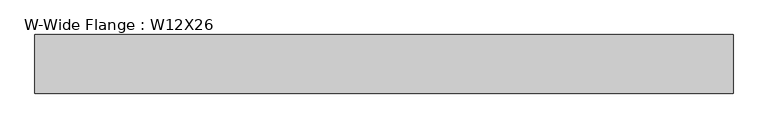
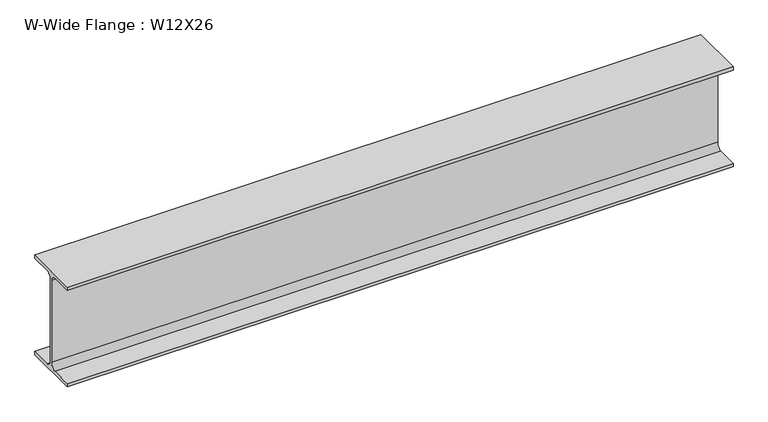
"""IFC4 building model written with IfcOpenShell, lengths in millimetres: beam geometry, W-Wide Flange : W12X26."""

from ifc_helpers import new_model, si_unit, point, frame, frame_2d, origin, place, context, project, spatial, polyline, circle_curve, trimmed, segment, composite_curve, outline, extrude, source, transform, mapped, element, save


def w_wide_flange_w12x26_057477a8(model_context):
    return source(origin(), model_context, "Body", "SweptSolid", [
        extrude(outline(composite_curve([segment(polyline([(-82.4011719, -145.5539063), (-20.2902344, -145.5539063)]), True, "CONTINUOUS"), segment(trimmed(circle_curve(frame_2d((-20.2902344, -128.190625)), 17.3632812), [point((-20.2902344, -145.5539063))], [point((-2.9269531, -128.190625))], True, "CARTESIAN"), True, "CONTINUOUS"), segment(polyline([(-2.9269531, -128.190625), (-2.9269531, 128.190625)]), True, "CONTINUOUS"), segment(trimmed(circle_curve(frame_2d((-20.2902344, 128.190625)), 17.3632812), [point((-2.9269531, 128.190625))], [point((-20.2902344, 145.5539062))], True, "CARTESIAN"), True, "CONTINUOUS"), segment(polyline([(-20.2902344, 145.5539062), (-82.4011719, 145.5539062), (-82.4011719, 155.178125), (82.4011719, 155.178125), (82.4011719, 145.5539062), (20.2902344, 145.5539062)]), True, "CONTINUOUS"), segment(trimmed(circle_curve(frame_2d((20.2902344, 128.190625)), 17.3632812), [point((20.2902344, 145.5539062))], [point((2.9269531, 128.190625))], True, "CARTESIAN"), True, "CONTINUOUS"), segment(polyline([(2.9269531, 128.190625), (2.9269531, -128.190625)]), True, "CONTINUOUS"), segment(trimmed(circle_curve(frame_2d((20.2902344, -128.190625)), 17.3632812), [point((2.9269531, -128.190625))], [point((20.2902344, -145.5539063))], True, "CARTESIAN"), True, "CONTINUOUS"), segment(polyline([(20.2902344, -145.5539063), (82.4011719, -145.5539063), (82.4011719, -155.178125), (-82.4011719, -155.178125), (-82.4011719, -145.5539063)]), True, "CONTINUOUS")], self_intersect=False)), frame((-984.25, 0.0, 0.0), z_axis=(1.0, 0.0, 0.0), x_axis=(0.0, 1.0, 0.0)), (0.0, 0.0, 1.0), 1962.15),
    ])


if __name__ == "__main__":
    model = new_model("IFC4")
    model_context = context("Model", 3, world=origin())
    ifc_project = project(units=[si_unit("LENGTHUNIT", "METRE", prefix="MILLI")], contexts=[model_context])
    site = spatial("IfcSite", under=ifc_project)
    building = spatial("IfcBuilding", under=site)
    placement = place(None, origin())
    w_wide_flange_w12x26_shape = w_wide_flange_w12x26_057477a8(model_context)
    element("IfcBeam", 1, ObjectType="W-Wide Flange : W12X26", at=placement, inside=building, context=model_context, shape_type="MappedRepresentation", body=[
        mapped(w_wide_flange_w12x26_shape, transform((0.0, 0.0, 0.0), x_axis=(1.0, 0.0, 0.0), y_axis=(0.0, 1.0, 0.0), z_axis=(0.0, 0.0, 1.0))),
    ])
    save(model, "model.ifc")

# Revit data of these elements
# Type "W-Wide Flange : W12X26"
#   Assembly Code = "B10"
#   W = 26
#   Start Extension Calculation [instance default] = 10' - 0"
#   Start Extension [instance default] = -0' - 0 1/2"
#   End Extension Calculation [instance default] = 10' - 0"
#   End Extension [instance default] = -0' - 0 1/2"
#   Length [instance default] = 5' - 0"
#   bf = 0' - 6 125/256"
#   d = 1' - 0 7/32"
#   k = 0' - 1 1/16"
#   k2 = 0' - 0 175/256"
#   tf = 0' - 0 97/256"
#   tw = 0' - 0 59/256"
#   A = 0.05 SF
#   Beam Material [instance default] = Metal - Steel - ASTM A992
# Element 1 (IfcBeam, "W-Wide Flange : W12X26")
#   Materials on its faces: "Metal - Steel - ASTM A992"
# Materials
#   "Metal - Steel - ASTM A992": class "Metal", colour RGB 128 0 0, transparency 0
